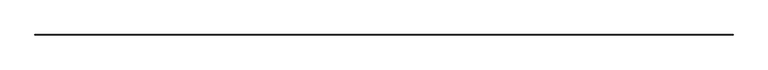
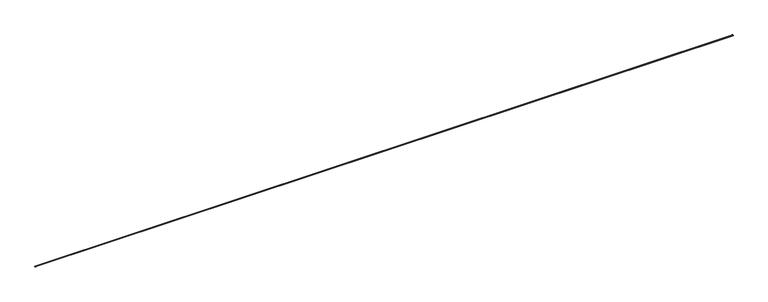
"""IFC4 building model written with IfcOpenShell, lengths in millimetres: proxy geometry, Generic Models 3:Generic Models 2:312240:Generic Models 2:312240 : Generic Models 3:Generic Models 2:312240:3 : Generic Models 3:Generic Models 2:312240:Generic Models 2:312240 : Generic Models 3:Generic Models 2:312240:300533."""

from ifc_helpers import new_model, si_unit, frame, origin, place, context, project, spatial, polyline, outline, extrude, source, transform, mapped, element, save


def generic_models_d9cae916(model_context):
    return source(origin(), model_context, "Body", "SweptSolid", [
        extrude(outline(polyline([(-568244.1474138, 4917.8153596), (-568244.0981692, 4916.8654907), (-568244.8387242, 4916.3717874), (-568245.8520509, 4917.0304498), (-568247.2599276, 4917.0304498), (-568247.2599276, 4914.7181249), (-568250.4023179, 4914.7181249), (-568250.4023179, 4979.2260614), (-568244.9476027, 4979.2260614), (-568244.9476027, 4976.0836711), (-568246.7263142, 4975.7872192), (-568244.9476027, 4970.9254078), (-568244.9476027, 4966.6565002), (-568247.2599276, 4966.6565002), (-568247.2599276, 4922.1294227), (-568235.1053992, 4922.1294227), (-568235.1053992, 4920.7572738), (-568245.0068931, 4919.3427747), (-568245.0068931, 4918.2919877), (-568244.1474138, 4917.8153596)])), frame((592424.3745369, 0.0, 0.0), z_axis=(1.0, 0.0, 0.0), x_axis=(0.0, 1.0, 0.0)), (0.0, 0.0, 1.0), 76828.8898905),
        extrude(outline(polyline([(-568248.7898792, 4980.4623942), (-568237.3584337, 4983.5107797), (-568237.3584337, 4971.9051667), (-568243.4517132, 4966.6565002), (-568244.6570171, 4966.6565002), (-568244.6570171, 4971.1856364), (-568246.199054, 4975.4005372), (-568244.6570171, 4975.6575433), (-568244.6570171, 4979.4237811), (-568248.7898792, 4979.4237811), (-568248.7898792, 4980.4623942)])), frame((592424.3745369, 0.0, 0.0), z_axis=(1.0, 0.0, 0.0), x_axis=(0.0, 1.0, 0.0)), (0.0, 0.0, 1.0), 76828.8898905),
        extrude(outline(polyline([(-568189.4518044, 4967.3679848), (-568194.0171639, 4967.3679848), (-568194.0171639, 4969.4135794), (-568192.7127754, 4970.7178519), (-568192.7127754, 4968.9095348), (-568191.2305159, 4968.9095348), (-568190.2366955, 4970.6308821), (-568190.2366955, 4972.9123012), (-568191.1221172, 4974.8110942), (-568192.7127754, 4974.8110942), (-568192.7127754, 4972.7778707), (-568194.0171639, 4973.0005712), (-568194.0171639, 4978.0402537), (-568186.9023179, 4977.4418087), (-568186.9023179, 4915.0145768), (-568190.4597409, 4915.0145768), (-568190.4597409, 4908.7297962), (-568192.4756139, 4908.7297962), (-568192.4756139, 4915.0145768), (-568203.3850443, 4915.0145768), (-568203.3850443, 4908.7297962), (-568205.4009174, 4908.7297962), (-568205.4009174, 4915.0145768), (-568236.469078, 4915.0145768), (-568236.469078, 4908.7297962), (-568238.484951, 4908.7297962), (-568238.484951, 4915.0145768), (-568247.0820565, 4915.0145768), (-568247.0820565, 4916.3782556), (-568246.2519911, 4916.911869), (-568245.303345, 4916.2596748), (-568238.484951, 4916.2596748), (-568237.1805626, 4917.5640632), (-568233.4452684, 4917.5640632), (-568233.4452684, 4922.9001977), (-568246.9041853, 4922.9001977), (-568246.9041853, 4924.4417476), (-568231.4293954, 4924.4417476), (-568231.4293954, 4917.5640632), (-568205.5194981, 4917.5640632), (-568205.5194981, 4924.4417476), (-568189.4518044, 4924.4417476), (-568189.4518044, 4967.3679848)]), holes=[polyline([(-568190.0447082, 4917.1490306), (-568190.0447082, 4922.9001977), (-568203.3850443, 4922.9001977), (-568203.3850443, 4917.1490306), (-568190.0447082, 4917.1490306)])]), frame((592424.3745369, 0.0, 0.0), z_axis=(1.0, 0.0, 0.0), x_axis=(0.0, 1.0, 0.0)), (0.0, 0.0, 1.0), 76828.8898905),
        extrude(outline(polyline([(-568197.3584337, 4982.0206037), (-568187.3997943, 4979.8018394), (-568187.3997943, 4977.7004245), (-568194.3240093, 4978.2828351), (-568194.3240093, 4972.8425353), (-568192.4003572, 4972.5141069), (-568192.4003572, 4974.5523703), (-568191.3760083, 4974.5523703), (-568190.5359627, 4972.7508867), (-568190.5359627, 4970.6705882), (-568191.396411, 4969.1802479), (-568192.4855979, 4969.1802479), (-568192.4855979, 4971.4346361), (-568194.3240093, 4969.5962247), (-568194.3240093, 4967.3679848), (-568197.3584337, 4967.3679848), (-568197.3584337, 4982.0206037)])), frame((592424.3745369, 0.0, 0.0), z_axis=(1.0, 0.0, 0.0), x_axis=(0.0, 1.0, 0.0)), (0.0, 0.0, 1.0), 76828.8898905),
    ])


if __name__ == "__main__":
    model = new_model("IFC4")
    model_context = context("Model", 3, world=origin())
    ifc_project = project(units=[si_unit("LENGTHUNIT", "METRE", prefix="MILLI")], contexts=[model_context])
    site = spatial("IfcSite", under=ifc_project)
    building = spatial("IfcBuilding", under=site)
    placement = place(None, origin())
    generic_models_shape = generic_models_d9cae916(model_context)
    element("IfcBuildingElementProxy", 1, Name="Generic Models 3:Generic Models 2:312240:Generic Models 2:312240 : Generic Models 3:Generic Models 2:312240:3 : Generic Models 3:Generic Models 2:312240:Generic Models 2:312240 : Generic Models 3:Generic Models 2:312240:300533", ObjectType="Generic Models 3:Generic Models 2:312240:Generic Models 2:312240 : Generic Models 3:Generic Models 2:312240:3 : Generic Models 3:Generic Models 2:312240:Generic Models 2:312240 : Generic Models 3:Generic Models 2:312240:300533", at=placement, inside=building, context=model_context, shape_type="MappedRepresentation", body=[
        mapped(generic_models_shape, transform((0.0, 0.0, 0.0), x_axis=(1.0, 0.0, 0.0), y_axis=(0.0, 1.0, 0.0), z_axis=(0.0, 0.0, 1.0))),
    ])
    save(model, "model.ifc")

# Revit data of these elements
# Type "Generic Models 3:Generic Models 2:312240:Generic Models 2:312240 : Generic Models 3:Generic Models 2:312240:3 : Generic Models 3:Generic Models 2:312240:Generic Models 2:312240 : Generic Models 3:Generic Models 2:312240:300533"
#   NameOverride = "Generic Models 3:Generic Models 2:312240:Generic Models 2:312240 : Generic Models 3:Generic Models 2:312240:300533"
#   ObjectTypeOverride = "Generic Models 2:312240 : Generic Models 3:Generic Models 2:312240"
#   Reference = "Generic Models 2"
#   Tag = "300533"
# Element 1 (IfcBuildingElementProxy, "Generic Models 3:Generic Models 2:312240:Generic Models 2:312240 : Generic Models 3:Generic Models 2:312240:3 : Generic Models 3:Generic Models 2:312240:Generic Models 2:312240 : Generic Models 3:Generic Models 2:312240:300533")
#   Materials on its faces: "THERMAL BROKEN ALUMINUM STOREFRONT FOR POLYCARBONATE"
# Materials
#   "THERMAL BROKEN ALUMINUM STOREFRONT FOR POLYCARBONATE": class "Unassigned", colour RGB 244 244 244, transparency 0, Keynote = "M07611300.01", Cost = 0
